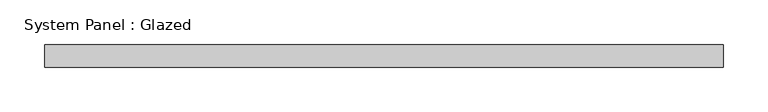
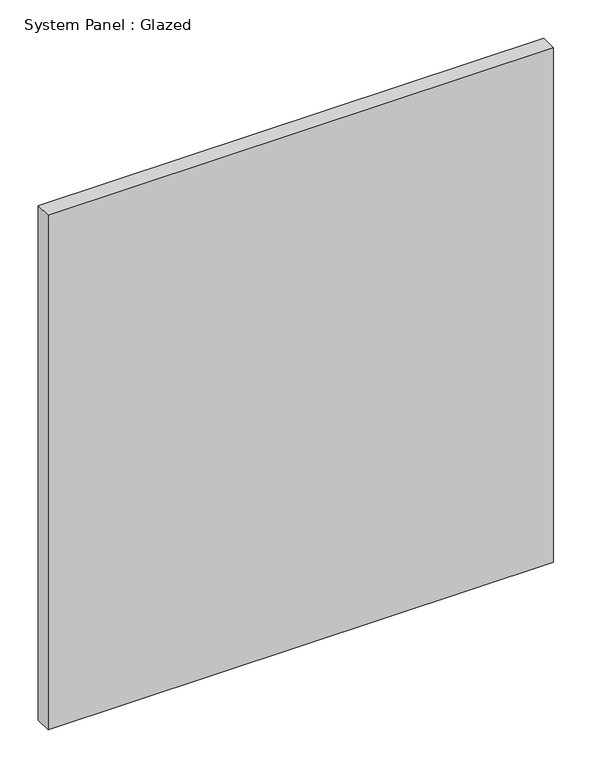
"""IFC4 building model written with IfcOpenShell, lengths in millimetres: plate geometry, System Panel : Glazed."""

import ifcopenshell
import ifcopenshell.guid

model = None  # the IFC model being written
_history = None  # IfcOwnerHistory: only IFC2X3 demands one
_inside = {}  # id of a spatial element -> (the spatial element, [elements in it])
_under = {}  # id of a project, library or spatial element -> (it, [spatial elements below it])
_declared = {}  # id of a project -> (the project, [libraries it declares])
_typed = {}  # id of a type object -> (the type object, [elements of that type])
_made_of = {}  # id of a material, layer set ... -> (it, [elements and type objects made of it])


def new_model(schema):
    """Start an empty IFC model of exactly this schema.

    Asked for "IFC4X3", IfcOpenShell would pick the latest addendum, in which some entities
    have other attributes; the version numbers below select the first issue.
    IFC2X3 requires an IfcOwnerHistory on every rooted entity: one is made here for all.
    """
    global model, _history
    if schema == "IFC4X3":
        model = ifcopenshell.file(schema_version=(4, 3, 0, 0))
    else:
        model = ifcopenshell.file(schema=schema)
    _inside.clear()
    _under.clear()
    _declared.clear()
    _typed.clear()
    _made_of.clear()
    _history = None
    if model.schema == "IFC2X3":
        org = make("IfcOrganization", Name="unknown")
        user = make(
            "IfcPersonAndOrganization",
            ThePerson=make("IfcPerson", FamilyName="unknown"),
            TheOrganization=org,
        )
        app = make(
            "IfcApplication",
            ApplicationDeveloper=org,
            Version="unknown",
            ApplicationFullName="unknown",
            ApplicationIdentifier="unknown",
        )
        _history = make(
            "IfcOwnerHistory",
            OwningUser=user,
            OwningApplication=app,
            ChangeAction="ADDED",
            CreationDate=0,
        )
    return model


def make(cls, **values):
    """One entity of the class cls with the attributes given. An attribute that is None is left unset."""
    return model.create_entity(
        cls, **{name: value for name, value in values.items() if value is not None}
    )


def rooted(cls, **values):
    """An entity with a GlobalId (a new one), such as an element, a storey or a relation."""
    return make(cls, GlobalId=ifcopenshell.guid.new(), OwnerHistory=_history, **values)


def si_unit(unit_type, name, prefix=None):
    """IfcSIUnit, for example si_unit("LENGTHUNIT", "METRE", prefix="MILLI")."""
    return make("IfcSIUnit", UnitType=unit_type, Prefix=prefix, Name=name)


def assignment(units):
    """IfcUnitAssignment: the units of a project."""
    return None if units is None else make("IfcUnitAssignment", Units=units)


def point(xyz):
    """IfcCartesianPoint."""
    return None if xyz is None else make("IfcCartesianPoint", Coordinates=xyz)


def direction(xyz):
    """IfcDirection."""
    return None if xyz is None else make("IfcDirection", DirectionRatios=xyz)


def frame(location, z_axis=None, x_axis=None):
    """IfcAxis2Placement3D, a coordinate frame: its origin and axes. An axis left out is left unset."""
    return make(
        "IfcAxis2Placement3D",
        Location=point(location),
        Axis=direction(z_axis),
        RefDirection=direction(x_axis),
    )


def origin():
    """The frame at (0, 0, 0) with its axes left unset."""
    return frame((0.0, 0.0, 0.0))


def origin_with_axes():
    """The frame at (0, 0, 0) with the z axis (0, 0, 1) and the x axis (1, 0, 0) written out."""
    return frame((0.0, 0.0, 0.0), z_axis=(0.0, 0.0, 1.0), x_axis=(1.0, 0.0, 0.0))


def place(relative_to, where):
    """IfcLocalPlacement: puts the frame where relative to a parent placement (None: the world)."""
    return make(
        "IfcLocalPlacement", PlacementRelTo=relative_to, RelativePlacement=where
    )


def context(
    kind, dimensions, precision=None, world=None, true_north=None, identifier=None
):
    """IfcGeometricRepresentationContext, for example the 3D "Model" context."""
    return make(
        "IfcGeometricRepresentationContext",
        ContextIdentifier=identifier,
        ContextType=kind,
        CoordinateSpaceDimension=dimensions,
        Precision=precision,
        WorldCoordinateSystem=world,
        TrueNorth=true_north,
    )


def project(units=None, contexts=None):
    """IfcProject with its units and contexts."""
    return rooted(
        "IfcProject",
        Name="project",
        RepresentationContexts=contexts,
        UnitsInContext=assignment(units),
    )


def spatial(cls, under=None, at=None, **own):
    """A site, building, storey or space (cls), placed at a placement, below another one or the project."""
    s = rooted(cls, ObjectPlacement=at, **own)
    if under is not None:
        _under.setdefault(under.id(), (under, []))[1].append(s)
    return s


def polyline(points):
    """IfcPolyline through the points."""
    return make("IfcPolyline", Points=[point(p) for p in points])


def outline(outer, holes=None, kind="AREA"):
    """IfcArbitraryClosedProfileDef: a profile drawn as a closed curve; with holes, ...WithVoids."""
    if holes is None:
        return make("IfcArbitraryClosedProfileDef", ProfileType=kind, OuterCurve=outer)
    return make(
        "IfcArbitraryProfileDefWithVoids",
        ProfileType=kind,
        OuterCurve=outer,
        InnerCurves=holes,
    )


def extrude(swept, where, along, depth):
    """IfcExtrudedAreaSolid: the profile swept, set in the frame where, extruded along a direction by depth."""
    return make(
        "IfcExtrudedAreaSolid",
        SweptArea=swept,
        Position=where,
        ExtrudedDirection=direction(along),
        Depth=depth,
    )


def shape(context_of_items, identifier, shape_type, items):
    """IfcShapeRepresentation: the items that make up one representation, for example the "Body"."""
    return make(
        "IfcShapeRepresentation",
        ContextOfItems=context_of_items,
        RepresentationIdentifier=identifier,
        RepresentationType=shape_type,
        Items=items,
    )


def source(mapping_origin, context_of_items, identifier, shape_type, items):
    """IfcRepresentationMap: a shape defined once, which mapped items show again and again."""
    return make(
        "IfcRepresentationMap",
        MappingOrigin=mapping_origin,
        MappedRepresentation=shape(context_of_items, identifier, shape_type, items),
    )


def transform(
    local_origin,
    x_axis=None,
    y_axis=None,
    z_axis=None,
    scale=None,
    scale2=None,
    scale3=None,
    uniform=True,
):
    """IfcCartesianTransformationOperator3D, or its non-uniform kind. x_axis, y_axis, z_axis: its Axis1, 2, 3."""
    if uniform:
        return make(
            "IfcCartesianTransformationOperator3D",
            Axis1=direction(x_axis),
            Axis2=direction(y_axis),
            LocalOrigin=point(local_origin),
            Scale=scale,
            Axis3=direction(z_axis),
        )
    return make(
        "IfcCartesianTransformationOperator3DnonUniform",
        Axis1=direction(x_axis),
        Axis2=direction(y_axis),
        LocalOrigin=point(local_origin),
        Scale=scale,
        Axis3=direction(z_axis),
        Scale2=scale2,
        Scale3=scale3,
    )


def mapped(mapping_source, mapping_target):
    """IfcMappedItem: shows the shape of a source again, moved by a transform."""
    return make(
        "IfcMappedItem", MappingSource=mapping_source, MappingTarget=mapping_target
    )


def made_of(thing, what):
    """Note that an element or type object is made of a material, layer set ...; save() writes the relation."""
    if what is not None:
        _made_of.setdefault(what.id(), (what, []))[1].append(thing)
    return thing


def element(
    cls,
    number,
    at=None,
    inside=None,
    cuts=None,
    type_object=None,
    material=None,
    context=None,
    identifier="Body",
    shape_type=None,
    held_by="IfcProductDefinitionShape",
    body=None,
    shapes=None,
    **own,
):
    """One element of the class cls, such as IfcWall. Its Tag is "e" and its number.

    at: its placement. inside: the storey or other place that contains it. cuts: it is an
    opening in that element (IfcRelVoidsElement). A single representation is given by context,
    identifier, shape_type and body (its items); several are given by shapes. held_by: the class
    of the entity that holds the representations. save() writes the other relations.
    """
    e = rooted(cls, Tag="e%d" % number, ObjectPlacement=at, **own)
    if body is not None:
        shapes = [shape(context, identifier, shape_type, body)]
    if shapes is not None:
        e.Representation = make(held_by, Representations=shapes)
    if inside is not None:
        _inside.setdefault(inside.id(), (inside, []))[1].append(e)
    if cuts is not None:
        rooted(
            "IfcRelVoidsElement", RelatingBuildingElement=cuts, RelatedOpeningElement=e
        )
    if type_object is not None:
        _typed.setdefault(type_object.id(), (type_object, []))[1].append(e)
    return made_of(e, material)


def aggregate(whole, parts):
    """IfcRelAggregates: a whole, such as a stair, and the parts it consists of."""
    return rooted("IfcRelAggregates", RelatingObject=whole, RelatedObjects=parts)


def save(model, path):
    """Write the relations noted so far, then the file.

    IfcRelAggregates (storeys below a building ...), IfcRelContainedInSpatialStructure (elements
    in a storey), IfcRelDefinesByType, IfcRelAssociatesMaterial and IfcRelDeclares: one each for
    every whole, place, type object, material and project.
    """
    for whole, parts in _under.values():
        aggregate(whole, parts)
    for where, things in _inside.values():
        rooted(
            "IfcRelContainedInSpatialStructure",
            RelatedElements=things,
            RelatingStructure=where,
        )
    for kind, things in _typed.values():
        rooted("IfcRelDefinesByType", RelatedObjects=things, RelatingType=kind)
    for what, things in _made_of.values():
        rooted("IfcRelAssociatesMaterial", RelatedObjects=things, RelatingMaterial=what)
    for by, libraries in _declared.values():
        rooted("IfcRelDeclares", RelatingContext=by, RelatedDefinitions=libraries)
    model.write(path)


def system_panel_glazed_99ba6c15(model_context):
    return source(origin(), model_context, "Body", "SweptSolid", [
        extrude(outline(polyline([(381.0, 19.05), (-381.0, 19.05), (-381.0, 44.45), (381.0, 44.45), (381.0, 19.05)])), origin_with_axes(), (0.0, 0.0, 1.0), 819.15),
    ])


if __name__ == "__main__":
    model = new_model("IFC4")
    model_context = context("Model", 3, world=origin())
    ifc_project = project(units=[si_unit("LENGTHUNIT", "METRE", prefix="MILLI")], contexts=[model_context])
    site = spatial("IfcSite", under=ifc_project)
    building = spatial("IfcBuilding", under=site)
    placement = place(None, origin())
    system_panel_glazed_shape = system_panel_glazed_99ba6c15(model_context)
    element("IfcPlate", 1, ObjectType="System Panel : Glazed", at=placement, inside=building, context=model_context, shape_type="MappedRepresentation", body=[
        mapped(system_panel_glazed_shape, transform((0.0, 0.0, 0.0), x_axis=(1.0, 0.0, 0.0), y_axis=(0.0, 1.0, 0.0), z_axis=(0.0, 0.0, 1.0))),
    ])
    save(model, "model.ifc")

# Revit data of these elements
# Type "System Panel : Glazed"
#   Construction Type Id = "GSP4R"
#   Analytic Construction = "1/8 in Pilkington single glazing"
#   Visual Light Transmittance = 0.9
#   Solar Heat Gain Coefficient = 0.86
#   Heat Transfer Coefficient (U) = 1.18115 BTU/(h·ft²·°F)
#   Define Thermal Properties by = 1
# Element 1 (IfcPlate, "System Panel : Glazed")
#   Materials on its faces: "Glass"
# Materials
#   "Glass": class "Glass", colour RGB 0 128 192, transparency 0.75, Description = "Soda Lime Glass", Cost = 0
